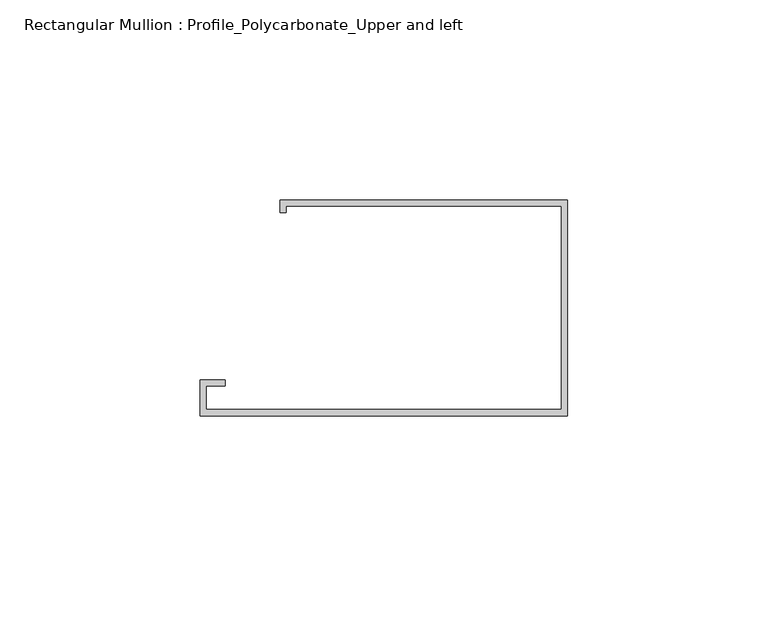
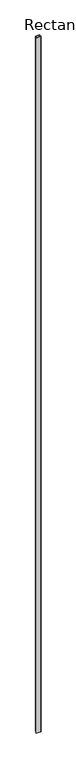
"""IFC4 building model written with IfcOpenShell, lengths in millimetres: member geometry, Rectangular Mullion : Profile_Polycarbonate_Upper and left."""

import ifcopenshell
import ifcopenshell.guid

model = None  # the IFC model being written
_history = None  # IfcOwnerHistory: only IFC2X3 demands one
_inside = {}  # id of a spatial element -> (the spatial element, [elements in it])
_under = {}  # id of a project, library or spatial element -> (it, [spatial elements below it])
_declared = {}  # id of a project -> (the project, [libraries it declares])
_typed = {}  # id of a type object -> (the type object, [elements of that type])
_made_of = {}  # id of a material, layer set ... -> (it, [elements and type objects made of it])


def new_model(schema):
    """Start an empty IFC model of exactly this schema.

    Asked for "IFC4X3", IfcOpenShell would pick the latest addendum, in which some entities
    have other attributes; the version numbers below select the first issue.
    IFC2X3 requires an IfcOwnerHistory on every rooted entity: one is made here for all.
    """
    global model, _history
    if schema == "IFC4X3":
        model = ifcopenshell.file(schema_version=(4, 3, 0, 0))
    else:
        model = ifcopenshell.file(schema=schema)
    _inside.clear()
    _under.clear()
    _declared.clear()
    _typed.clear()
    _made_of.clear()
    _history = None
    if model.schema == "IFC2X3":
        org = make("IfcOrganization", Name="unknown")
        user = make(
            "IfcPersonAndOrganization",
            ThePerson=make("IfcPerson", FamilyName="unknown"),
            TheOrganization=org,
        )
        app = make(
            "IfcApplication",
            ApplicationDeveloper=org,
            Version="unknown",
            ApplicationFullName="unknown",
            ApplicationIdentifier="unknown",
        )
        _history = make(
            "IfcOwnerHistory",
            OwningUser=user,
            OwningApplication=app,
            ChangeAction="ADDED",
            CreationDate=0,
        )
    return model


def make(cls, **values):
    """One entity of the class cls with the attributes given. An attribute that is None is left unset."""
    return model.create_entity(
        cls, **{name: value for name, value in values.items() if value is not None}
    )


def rooted(cls, **values):
    """An entity with a GlobalId (a new one), such as an element, a storey or a relation."""
    return make(cls, GlobalId=ifcopenshell.guid.new(), OwnerHistory=_history, **values)


def si_unit(unit_type, name, prefix=None):
    """IfcSIUnit, for example si_unit("LENGTHUNIT", "METRE", prefix="MILLI")."""
    return make("IfcSIUnit", UnitType=unit_type, Prefix=prefix, Name=name)


def assignment(units):
    """IfcUnitAssignment: the units of a project."""
    return None if units is None else make("IfcUnitAssignment", Units=units)


def point(xyz):
    """IfcCartesianPoint."""
    return None if xyz is None else make("IfcCartesianPoint", Coordinates=xyz)


def direction(xyz):
    """IfcDirection."""
    return None if xyz is None else make("IfcDirection", DirectionRatios=xyz)


def frame(location, z_axis=None, x_axis=None):
    """IfcAxis2Placement3D, a coordinate frame: its origin and axes. An axis left out is left unset."""
    return make(
        "IfcAxis2Placement3D",
        Location=point(location),
        Axis=direction(z_axis),
        RefDirection=direction(x_axis),
    )


def origin():
    """The frame at (0, 0, 0) with its axes left unset."""
    return frame((0.0, 0.0, 0.0))


def place(relative_to, where):
    """IfcLocalPlacement: puts the frame where relative to a parent placement (None: the world)."""
    return make(
        "IfcLocalPlacement", PlacementRelTo=relative_to, RelativePlacement=where
    )


def context(
    kind, dimensions, precision=None, world=None, true_north=None, identifier=None
):
    """IfcGeometricRepresentationContext, for example the 3D "Model" context."""
    return make(
        "IfcGeometricRepresentationContext",
        ContextIdentifier=identifier,
        ContextType=kind,
        CoordinateSpaceDimension=dimensions,
        Precision=precision,
        WorldCoordinateSystem=world,
        TrueNorth=true_north,
    )


def project(units=None, contexts=None):
    """IfcProject with its units and contexts."""
    return rooted(
        "IfcProject",
        Name="project",
        RepresentationContexts=contexts,
        UnitsInContext=assignment(units),
    )


def spatial(cls, under=None, at=None, **own):
    """A site, building, storey or space (cls), placed at a placement, below another one or the project."""
    s = rooted(cls, ObjectPlacement=at, **own)
    if under is not None:
        _under.setdefault(under.id(), (under, []))[1].append(s)
    return s


def polyline(points):
    """IfcPolyline through the points."""
    return make("IfcPolyline", Points=[point(p) for p in points])


def outline(outer, holes=None, kind="AREA"):
    """IfcArbitraryClosedProfileDef: a profile drawn as a closed curve; with holes, ...WithVoids."""
    if holes is None:
        return make("IfcArbitraryClosedProfileDef", ProfileType=kind, OuterCurve=outer)
    return make(
        "IfcArbitraryProfileDefWithVoids",
        ProfileType=kind,
        OuterCurve=outer,
        InnerCurves=holes,
    )


def extrude(swept, where, along, depth):
    """IfcExtrudedAreaSolid: the profile swept, set in the frame where, extruded along a direction by depth."""
    return make(
        "IfcExtrudedAreaSolid",
        SweptArea=swept,
        Position=where,
        ExtrudedDirection=direction(along),
        Depth=depth,
    )


def shape(context_of_items, identifier, shape_type, items):
    """IfcShapeRepresentation: the items that make up one representation, for example the "Body"."""
    return make(
        "IfcShapeRepresentation",
        ContextOfItems=context_of_items,
        RepresentationIdentifier=identifier,
        RepresentationType=shape_type,
        Items=items,
    )


def source(mapping_origin, context_of_items, identifier, shape_type, items):
    """IfcRepresentationMap: a shape defined once, which mapped items show again and again."""
    return make(
        "IfcRepresentationMap",
        MappingOrigin=mapping_origin,
        MappedRepresentation=shape(context_of_items, identifier, shape_type, items),
    )


def transform(
    local_origin,
    x_axis=None,
    y_axis=None,
    z_axis=None,
    scale=None,
    scale2=None,
    scale3=None,
    uniform=True,
):
    """IfcCartesianTransformationOperator3D, or its non-uniform kind. x_axis, y_axis, z_axis: its Axis1, 2, 3."""
    if uniform:
        return make(
            "IfcCartesianTransformationOperator3D",
            Axis1=direction(x_axis),
            Axis2=direction(y_axis),
            LocalOrigin=point(local_origin),
            Scale=scale,
            Axis3=direction(z_axis),
        )
    return make(
        "IfcCartesianTransformationOperator3DnonUniform",
        Axis1=direction(x_axis),
        Axis2=direction(y_axis),
        LocalOrigin=point(local_origin),
        Scale=scale,
        Axis3=direction(z_axis),
        Scale2=scale2,
        Scale3=scale3,
    )


def mapped(mapping_source, mapping_target):
    """IfcMappedItem: shows the shape of a source again, moved by a transform."""
    return make(
        "IfcMappedItem", MappingSource=mapping_source, MappingTarget=mapping_target
    )


def made_of(thing, what):
    """Note that an element or type object is made of a material, layer set ...; save() writes the relation."""
    if what is not None:
        _made_of.setdefault(what.id(), (what, []))[1].append(thing)
    return thing


def element(
    cls,
    number,
    at=None,
    inside=None,
    cuts=None,
    type_object=None,
    material=None,
    context=None,
    identifier="Body",
    shape_type=None,
    held_by="IfcProductDefinitionShape",
    body=None,
    shapes=None,
    **own,
):
    """One element of the class cls, such as IfcWall. Its Tag is "e" and its number.

    at: its placement. inside: the storey or other place that contains it. cuts: it is an
    opening in that element (IfcRelVoidsElement). A single representation is given by context,
    identifier, shape_type and body (its items); several are given by shapes. held_by: the class
    of the entity that holds the representations. save() writes the other relations.
    """
    e = rooted(cls, Tag="e%d" % number, ObjectPlacement=at, **own)
    if body is not None:
        shapes = [shape(context, identifier, shape_type, body)]
    if shapes is not None:
        e.Representation = make(held_by, Representations=shapes)
    if inside is not None:
        _inside.setdefault(inside.id(), (inside, []))[1].append(e)
    if cuts is not None:
        rooted(
            "IfcRelVoidsElement", RelatingBuildingElement=cuts, RelatedOpeningElement=e
        )
    if type_object is not None:
        _typed.setdefault(type_object.id(), (type_object, []))[1].append(e)
    return made_of(e, material)


def aggregate(whole, parts):
    """IfcRelAggregates: a whole, such as a stair, and the parts it consists of."""
    return rooted("IfcRelAggregates", RelatingObject=whole, RelatedObjects=parts)


def save(model, path):
    """Write the relations noted so far, then the file.

    IfcRelAggregates (storeys below a building ...), IfcRelContainedInSpatialStructure (elements
    in a storey), IfcRelDefinesByType, IfcRelAssociatesMaterial and IfcRelDeclares: one each for
    every whole, place, type object, material and project.
    """
    for whole, parts in _under.values():
        aggregate(whole, parts)
    for where, things in _inside.values():
        rooted(
            "IfcRelContainedInSpatialStructure",
            RelatedElements=things,
            RelatingStructure=where,
        )
    for kind, things in _typed.values():
        rooted("IfcRelDefinesByType", RelatedObjects=things, RelatingType=kind)
    for what, things in _made_of.values():
        rooted("IfcRelAssociatesMaterial", RelatedObjects=things, RelatingMaterial=what)
    for by, libraries in _declared.values():
        rooted("IfcRelDeclares", RelatingContext=by, RelatedDefinitions=libraries)
    model.write(path)


def rectangular_mullion_profile_polycarbonate_upper_and_left_f30dcdf4(model_context):
    return source(origin(), model_context, "Body", "SweptSolid", [
        extrude(outline(polyline([(0.0, -28.984575), (-91.9988, -28.984575), (-91.9988, -19.992975), (-85.6488, -19.992975), (-85.6488, -21.580475), (-90.4113, -21.580475), (-90.4113, -27.397075), (-1.5875, -27.397075), (-1.5875, 23.428325), (-70.3961, 23.428325), (-70.3961, 21.840825), (-71.9836, 21.840825), (-71.9836, 25.015825), (0.0, 25.015825), (0.0, -28.984575)])), frame((0.0, 0.0, -14432.1149), z_axis=(0.0, 0.0, 1.0), x_axis=(1.0, 0.0, 0.0)), (0.0, 0.0, 1.0), 14432.1149),
    ])


if __name__ == "__main__":
    model = new_model("IFC4")
    model_context = context("Model", 3, world=origin())
    ifc_project = project(units=[si_unit("LENGTHUNIT", "METRE", prefix="MILLI")], contexts=[model_context])
    site = spatial("IfcSite", under=ifc_project)
    building = spatial("IfcBuilding", under=site)
    placement = place(None, origin())
    rectangular_mullion_profile_polycarbonate_upper_and_left_shape = rectangular_mullion_profile_polycarbonate_upper_and_left_f30dcdf4(model_context)
    element("IfcMember", 1, ObjectType="Rectangular Mullion : Profile_Polycarbonate_Upper and left", at=placement, inside=building, context=model_context, shape_type="MappedRepresentation", body=[
        mapped(rectangular_mullion_profile_polycarbonate_upper_and_left_shape, transform((0.0, 0.0, 0.0), x_axis=(1.0, 0.0, 0.0), y_axis=(0.0, 1.0, 0.0), z_axis=(0.0, 0.0, 1.0))),
    ])
    save(model, "model.ifc")

# Revit data of these elements
# Type "Rectangular Mullion : Profile_Polycarbonate_Upper and left"
#   built-in parameter 1007322 = 0.177167 (stored number, unit not read)
#   built-in parameter 1007321 = 0.00520833 (stored number, unit not read)
#   built-in parameter 1007320 = 0 (stored number, unit not read)
